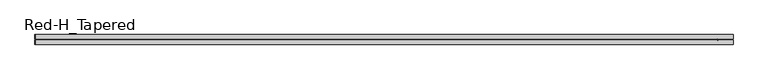
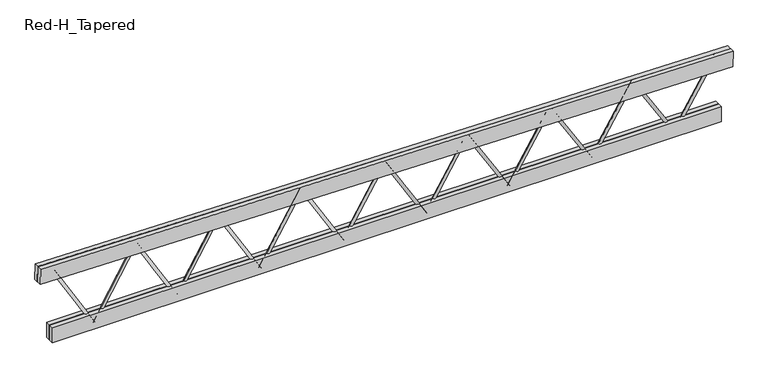
"""IFC4 building model written with IfcOpenShell, lengths in millimetres: beam geometry, Construction_Frames_RedBuilt_Openweb_Red-H_Tapered : Red-H_Tapered."""

from ifc_helpers import new_model, si_unit, point, frame, origin, origin_2d, place, context, project, spatial, polyline, circle_curve, trimmed, segment, composite_curve, outline, extrude, source, transform, mapped, element, save


def red_h_tapered_5ce7bd37(model_context):
    return source(origin(), model_context, "Body", "SweptSolid", [
        extrude(outline(composite_curve([segment(trimmed(circle_curve(origin_2d(), 12.7), [point((0.0, 12.7))], [point((0.0, -12.7))], False, "CARTESIAN"), True, "CONTINUOUS"), segment(trimmed(circle_curve(origin_2d(), 12.7), [point((0.0, -12.7))], [point((0.0, 12.7))], False, "CARTESIAN"), True, "CONTINUOUS")], self_intersect=False)), frame((2516.6154336, 0.0, -367.0101562), z_axis=(0.5241067286958753, 0.0, 0.8516525916920046), x_axis=(0.0, -1.0, 0.0)), (0.0, 0.0, 1.0), 685.9604558),
        extrude(outline(composite_curve([segment(trimmed(circle_curve(origin_2d(), 12.7), [point((0.0, -12.7))], [point((0.0, 12.6999999))], False, "CARTESIAN"), True, "CONTINUOUS"), segment(trimmed(circle_curve(origin_2d(), 12.7), [point((0.0, 12.6999999))], [point((0.0, -12.7))], False, "CARTESIAN"), True, "CONTINUOUS")], self_intersect=False)), frame((2516.6154336, 0.0, -367.0101562), z_axis=(-0.5215353438102012, 0.0, 0.853229679017775), x_axis=(0.0, -1.0, 0.0)), (0.0, 0.0, 1.0), 689.3425245),
        extrude(outline(composite_curve([segment(trimmed(circle_curve(origin_2d(), 12.7), [point((0.0, 12.7))], [point((0.0, -12.6999999))], False, "CARTESIAN"), True, "CONTINUOUS"), segment(trimmed(circle_curve(origin_2d(), 12.7), [point((0.0, -12.6999999))], [point((0.0, 12.7))], False, "CARTESIAN"), True, "CONTINUOUS")], self_intersect=False)), frame((1797.5824526, 0.0, -367.0101562), z_axis=(0.5215353438102003, 0.0, 0.8532296790177755), x_axis=(0.0, -1.0, 0.0)), (0.0, 0.0, 1.0), 689.3425245),
        extrude(outline(composite_curve([segment(trimmed(circle_curve(origin_2d(), 12.7), [point((0.0, -12.7))], [point((0.0, 12.7))], False, "CARTESIAN"), True, "CONTINUOUS"), segment(trimmed(circle_curve(origin_2d(), 12.7), [point((0.0, 12.7))], [point((0.0, -12.7))], False, "CARTESIAN"), True, "CONTINUOUS")], self_intersect=False)), frame((1797.5824526, 0.0, -367.0101562), z_axis=(-0.5189844139237941, 0.0, 0.8547837025260694), x_axis=(0.0, -1.0, 0.0)), (0.0, 0.0, 1.0), 692.7308044),
        extrude(outline(composite_curve([segment(trimmed(circle_curve(origin_2d(), 12.7), [point((0.0, 12.7000001))], [point((0.0, -12.7))], False, "CARTESIAN"), True, "CONTINUOUS"), segment(trimmed(circle_curve(origin_2d(), 12.7), [point((0.0, -12.7))], [point((0.0, 12.7000001))], False, "CARTESIAN"), True, "CONTINUOUS")], self_intersect=False)), frame((1078.5494715, 0.0, -367.0101562), z_axis=(0.518984413923793, 0.0, 0.8547837025260702), x_axis=(0.0, -1.0, 0.0)), (0.0, 0.0, 1.0), 692.7308044),
        extrude(outline(composite_curve([segment(trimmed(circle_curve(origin_2d(), 12.7), [point((0.0, -12.7))], [point((0.0, 12.7))], False, "CARTESIAN"), True, "CONTINUOUS"), segment(trimmed(circle_curve(origin_2d(), 12.7), [point((0.0, 12.7))], [point((0.0, -12.7))], False, "CARTESIAN"), True, "CONTINUOUS")], self_intersect=False)), frame((1078.5494715, 0.0, -367.0101562), z_axis=(-0.5164537759218651, 0.0, 0.856315068964717), x_axis=(0.0, -1.0, 0.0)), (0.0, 0.0, 1.0), 696.1252048),
        extrude(outline(composite_curve([segment(trimmed(circle_curve(origin_2d(), 12.7), [point((0.0, 12.7))], [point((0.0, -12.7))], False, "CARTESIAN"), True, "CONTINUOUS"), segment(trimmed(circle_curve(origin_2d(), 12.7), [point((0.0, -12.7))], [point((0.0, 12.7))], False, "CARTESIAN"), True, "CONTINUOUS")], self_intersect=False)), frame((359.5164905, 0.0, -367.0101562), z_axis=(0.5164537759218657, 0.0, 0.8563150689647167), x_axis=(0.0, -1.0, 0.0)), (0.0, 0.0, 1.0), 696.1252048),
        extrude(outline(composite_curve([segment(trimmed(circle_curve(origin_2d(), 12.7), [point((0.0, -12.7))], [point((0.0, 12.7))], False, "CARTESIAN"), True, "CONTINUOUS"), segment(trimmed(circle_curve(origin_2d(), 12.7), [point((0.0, 12.7))], [point((0.0, -12.7))], False, "CARTESIAN"), True, "CONTINUOUS")], self_intersect=False)), frame((359.5164905, 0.0, -367.0101562), z_axis=(-0.5139432662956527, 0.0, 0.8578241772236056), x_axis=(0.0, -1.0, 0.0)), (0.0, 0.0, 1.0), 699.5256366),
        extrude(outline(composite_curve([segment(trimmed(circle_curve(origin_2d(), 12.7), [point((0.0, -12.7))], [point((0.0, 12.7))], False, "CARTESIAN"), True, "CONTINUOUS"), segment(trimmed(circle_curve(origin_2d(), 12.7), [point((0.0, 12.7))], [point((0.0, -12.7))], False, "CARTESIAN"), True, "CONTINUOUS")], self_intersect=False)), frame((-359.5164905, 0.0, -367.0101562), z_axis=(0.5139432662956213, 0.0, 0.8578241772236244), x_axis=(0.0, -1.0, 0.0)), (0.0, 0.0, 1.0), 699.5256366),
        extrude(outline(composite_curve([segment(trimmed(circle_curve(origin_2d(), 12.7), [point((0.0, 12.7))], [point((0.0, -12.7))], False, "CARTESIAN"), True, "CONTINUOUS"), segment(trimmed(circle_curve(origin_2d(), 12.7), [point((0.0, -12.7))], [point((0.0, 12.7))], False, "CARTESIAN"), True, "CONTINUOUS")], self_intersect=False)), frame((-359.5164905, 0.0, -367.0101562), z_axis=(-0.511452721242837, 0.0, 0.8593114184818545), x_axis=(0.0, -1.0, 0.0)), (0.0, 0.0, 1.0), 702.9320123),
        extrude(outline(composite_curve([segment(trimmed(circle_curve(origin_2d(), 12.7), [point((0.0, -12.7))], [point((0.0, 12.7))], False, "CARTESIAN"), True, "CONTINUOUS"), segment(trimmed(circle_curve(origin_2d(), 12.7), [point((0.0, 12.7))], [point((0.0, -12.7))], False, "CARTESIAN"), True, "CONTINUOUS")], self_intersect=False)), frame((-1078.5494715, 0.0, -367.0101562), z_axis=(0.5114527212428354, 0.0, 0.8593114184818554), x_axis=(0.0, -1.0, 0.0)), (0.0, 0.0, 1.0), 702.9320123),
        extrude(outline(composite_curve([segment(trimmed(circle_curve(origin_2d(), 12.7), [point((0.0, 12.7))], [point((0.0, -12.7000001))], False, "CARTESIAN"), True, "CONTINUOUS"), segment(trimmed(circle_curve(origin_2d(), 12.7), [point((0.0, -12.7000001))], [point((0.0, 12.7))], False, "CARTESIAN"), True, "CONTINUOUS")], self_intersect=False)), frame((-1078.5494715, 0.0, -367.0101562), z_axis=(-0.5089819767631879, 0.0, 0.8607771763529966), x_axis=(0.0, -1.0, 0.0)), (0.0, 0.0, 1.0), 706.3442458),
        extrude(outline(composite_curve([segment(trimmed(circle_curve(origin_2d(), 12.7), [point((0.0, -12.7))], [point((0.0, 12.7000001))], False, "CARTESIAN"), True, "CONTINUOUS"), segment(trimmed(circle_curve(origin_2d(), 12.7), [point((0.0, 12.7000001))], [point((0.0, -12.7))], False, "CARTESIAN"), True, "CONTINUOUS")], self_intersect=False)), frame((-1797.5824526, 0.0, -367.0101562), z_axis=(0.508981976763201, 0.0, 0.8607771763529889), x_axis=(0.0, -1.0, 0.0)), (0.0, 0.0, 1.0), 706.3442458),
        extrude(outline(composite_curve([segment(trimmed(circle_curve(origin_2d(), 12.7), [point((0.0, 12.7))], [point((0.0, -12.7))], False, "CARTESIAN"), True, "CONTINUOUS"), segment(trimmed(circle_curve(origin_2d(), 12.7), [point((0.0, -12.7))], [point((0.0, 12.7))], False, "CARTESIAN"), True, "CONTINUOUS")], self_intersect=False)), frame((-1797.5824526, 0.0, -367.0101562), z_axis=(-0.5065308687490784, 0.0, 0.8622218270284648), x_axis=(0.0, -1.0, 0.0)), (0.0, 0.0, 1.0), 709.7622528),
        extrude(outline(composite_curve([segment(trimmed(circle_curve(origin_2d(), 12.7), [point((0.0, -12.7))], [point((0.0, 12.7))], False, "CARTESIAN"), True, "CONTINUOUS"), segment(trimmed(circle_curve(origin_2d(), 12.7), [point((0.0, 12.7))], [point((0.0, -12.7))], False, "CARTESIAN"), True, "CONTINUOUS")], self_intersect=False)), frame((-2516.6154336, 0.0, -367.0101562), z_axis=(0.5065308687490667, 0.0, 0.8622218270284718), x_axis=(0.0, -1.0, 0.0)), (0.0, 0.0, 1.0), 709.7622528),
        extrude(outline(composite_curve([segment(trimmed(circle_curve(origin_2d(), 12.7), [point((0.0, 12.7))], [point((0.0, -12.7))], False, "CARTESIAN"), True, "CONTINUOUS"), segment(trimmed(circle_curve(origin_2d(), 12.7), [point((0.0, -12.7))], [point((0.0, 12.7))], False, "CARTESIAN"), True, "CONTINUOUS")], self_intersect=False)), frame((-2516.6154336, 0.0, -367.0101562), z_axis=(-0.5040992330715739, 0.0, 0.8636457394190346), x_axis=(0.0, -1.0, 0.0)), (0.0, 0.0, 1.0), 713.1859502),
        extrude(outline(polyline([(-2901.5319241, -41.275), (-2901.5319241, -3.175), (2901.5319241, -3.175), (2901.5319241, -41.275), (-2901.5319241, -41.275)])), frame((0.0, 0.0, -386.0601562), z_axis=(0.0, 0.0, 1.0), x_axis=(1.0, 0.0, 0.0)), (0.0, 0.0, 1.0), 139.7),
        extrude(outline(polyline([(-2901.5319241, 3.175), (-2901.5319241, 41.275), (2901.5319241, 41.275), (2901.5319241, 3.175), (-2901.5319241, 3.175)])), frame((0.0, 0.0, -386.0601562), z_axis=(0.0, 0.0, 1.0), x_axis=(1.0, 0.0, 0.0)), (0.0, 0.0, 1.0), 139.7),
        extrude(outline(polyline([(0.0, -38.1), (0.0, 0.0), (6007.123103, 0.0), (6007.123103, -38.1), (0.0, -38.1)])), frame((-3005.4947057, -3.175, 185.4598263), z_axis=(0.016913254191312635, 0.0, 0.9998569606862074), x_axis=(0.9998569606862074, 0.0, -0.016913254191312635)), (0.0, 0.0, 1.0), 139.7),
        extrude(outline(polyline([(0.0, -38.1), (0.0, 0.0), (6007.123103, 0.0), (6007.123103, -38.1), (0.0, -38.1)])), frame((-3005.4947057, 41.275, 185.4598263), z_axis=(0.016913254191312635, 0.0, 0.9998569606862074), x_axis=(0.9998569606862074, 0.0, -0.016913254191312635)), (0.0, 0.0, 1.0), 139.7),
    ])


if __name__ == "__main__":
    model = new_model("IFC4")
    model_context = context("Model", 3, world=origin())
    ifc_project = project(units=[si_unit("LENGTHUNIT", "METRE", prefix="MILLI")], contexts=[model_context])
    site = spatial("IfcSite", under=ifc_project)
    building = spatial("IfcBuilding", under=site)
    placement = place(None, origin())
    red_h_tapered_shape = red_h_tapered_5ce7bd37(model_context)
    element("IfcBeam", 1, ObjectType="Construction_Frames_RedBuilt_Openweb_Red-H_Tapered : Red-H_Tapered", at=placement, inside=building, context=model_context, shape_type="MappedRepresentation", body=[
        mapped(red_h_tapered_shape, transform((0.0, 0.0, 0.0), x_axis=(1.0, 0.0, 0.0), y_axis=(0.0, 1.0, 0.0), z_axis=(0.0, 0.0, 1.0))),
    ])
    save(model, "model.ifc")

# Revit data of these elements
# Type "Construction_Frames_RedBuilt_Openweb_Red-H_Tapered : Red-H_Tapered"
#   Youtube clip = ""
#   Weight Net (Kg) = "0"
#   Webs = "Up to 2\" diameter tubular steel"
#   Uniformat II Description = ""
#   Uniformat II Code = ""
#   Uniclass 2015 Name = "Softwood trusses"
#   Uniclass 2015 Code = "Pr_20_85_90_81"
#   Uniclass 2.0 Description = "Structural Framing Systems"
#   Uniclass 2.0 Code = "SS-15-10-75"
#   Uniclass 1.4 Description = "Trusses"
#   Uniclass 1.4 Code = "L3523"
#   UNSPSC Code = "30103606"
#   Technical description = "http://www.redbuilt.com/reference/literature-and-other-resources"
#   Region South America = "None"
#   Region Oceania = "None"
#   Region North America = "US"
#   Region Middle East = "None"
#   Region Europe = "None"
#   Region Asia = "None"
#   Region Antarctica = "None"
#   Region Africa = "None"
#   QR code = "http://bimobject.com/redbuilt/product/redbuilt-0003"
#   Product url = "http://www.redbuilt.com/products/default.aspx?id=2"
#   Product group = "Wood Trusses"
#   Product family = "Construction"
#   Product data url = "https://bimobject.com/redbuilt/product/redbuilt-0003"
#   Product certification = ""
#   Product SKU = "redbuilt-0003"
#   Product Page URL = "http://www.redbuilt.com/commercial-systems/red-m-red-h-open-web-trusses"
#   Product Guid = "2c5793f2-6ffb-4665-b825-cf90c048e711"
#   Product Documentation Link = "http://www.redbuilt.com/documents/OW_Guide_2017_07_LowRes_wLinks.pdf"
#   OmniClass Description = "Wood Trusses"
#   OmniClass Code = "23-13 35 19 13 17"
#   NBS Reference Description = ""
#   NBS Reference Code = ""
#   Material secondary = "Steel"
#   Material main = "CHARRED WOOD"
#   Masterformat 2014 Description = "Metal-Web Wood Joists"
#   Masterformat 2014 Code = "06 17 36"
#   Manufacturer name = "RedBuilt"
#   Manufacturer country = "United States"
#   Installation instructions = "http://www.redbuilt.com/documents/Installation_Sheets_Open-Web.pdf"
#   IFC Classification = ""
#   EAN code = ""
#   Design country = "United States"
#   Product Information = "http://redbuilt.com/products/default.aspx?id=2"
#   Model = "Red-H-Tapered"
#   Manufacturer URL = "http://redbuilt.com/"
#   Manufacturer = "RedBuilt™"
#   Description = "Open Web Truss"
#   Date of publishing = "8/17/2010"
#   Contact us = "http://redbuilt.com/contact/"
#   Chords = "Double 1½\" x 5½\" MSR lumber"
#   COBIe Type Category = ""
#   Brand url = "http://www.redbuilt.com"
#   BIMobject main category code = "construction"
#   BIMobject main category = "Construction"
#   BIMobject category code = "construction-frames-trusses"
#   BIMobject category = "Frames & Trusses"
#   Web Radius = 0' - 0 1/2"
#   Web Layout Offset Start [instance default] = 0' - 5"
#   Web Layout Offset End [instance default] = 0' - 5"
#   Web Diameter = 0' - 1"
#   TotalLength [instance default] = 20' - 0"
#   Span Minimum = 4' - 0"
#   Span Maximum = 70' - 0"
#   Span Limit [instance default] = 20' - 0"
#   Nominal width = 0' - 0"
#   Nominal height = 0' - 0"
#   Inner Depth Top [instance default] = 0' - 2.76372"
#   Depth Start [instance default] = 6' - 0"
#   Top Chord Length [instance default] = 20' - 1.19701"
#   TC Extension Start Aux [instance default] = 0' - 0"
#   TC Extension End Aux [instance default] = 0' - 0"
#   T-B Chord Length Difference L [instance default] = 0' - 4"
#   T-B Chord Length Difference [instance default] = 0' - 4"
#   Height 2 [instance default] = 6' - 0"
#   Depth Minimum at Wall = 2' - 0"
#   Depth Maximum at Wall = 6' - 0"
#   Depth Lower End [instance default] = 2' - 0"
#   Depth Higher End [instance default] = 6' - 0"
#   Depth End [instance default] = 2' - 0"
#   Depth 2 [instance default] = 2' - 0"
#   Chord Width = 0' - 3 1/4"
#   Chord Thickness = 0' - 1 1/2"
#   Chord Depth = 0' - 5 1/2"
#   Offset Start [instance default] = 0' - 0"
#   TC Extension Start [instance default] = 0' - 0"
#   End Panel = 0' - 5"
#   Offset End [instance default] = 0' - 0"
#   TC Extension End [instance default] = 0' - 0"
#   Length [instance default] = 20' - 0"
#   Angle [instance default] = 5.71059°
#   Span Limit Warning [instance default] = no
#   Edition number = 1
#   Top Bearing Start [instance default] = yes
#   Top Bearing End [instance default] = yes
#   Bottom Bearing Start [instance default] = no
#   Bottom Bearing End [instance default] = no
#   8 Panels [instance default] = yes
#   16 Panels [instance default] = no
#   12 Panels [instance default] = no
#   Web Material = RedBuilt-Steel, Galvanized
#   Clip Material = RedBuilt-Steel, Galvanized
#   Chords Material = WOOD-OAKFIRE
#   URL = ""
#   Assembly Code = ""
# Element 1 (IfcBeam, "Construction_Frames_RedBuilt_Openweb_Red-H_Tapered : Red-H_Tapered")
#   TotalLength = 19' - 8.46708"
#   Span Limit = 19' - 8.46708"
#   Inner Depth Top = 0' - 2.75039"
#   Depth Start = 5' - 0"
#   Top Chord Length = 19' - 8.50091"
#   Height 2 = 5' - 0"
#   Depth Higher End = 5' - 0"
#   Depth 2 = 0' - 4"
#   Angle = 0.969104°
#   Materials on its faces: "RedBuilt-Steel, Galvanized", "WOOD-OAKFIRE"
# Materials
#   "RedBuilt-Steel, Galvanized": class "Metal", colour RGB 164 172 176, transparency 0, Manufacturer = "RedBuilt. LLC", Comments = "Openweb Metal Web", URL = "http://www.redbuilt.com/", Description = "Galvanized steel", Cost = 0
#   "WOOD-OAKFIRE": class "Wood", colour RGB 198 202 183, transparency 0, Description = "Generic wood", Cost = 0
